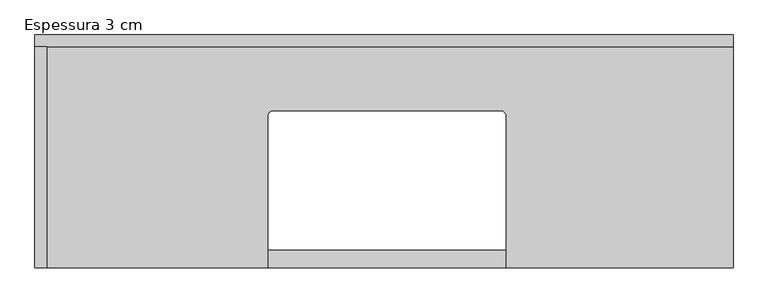
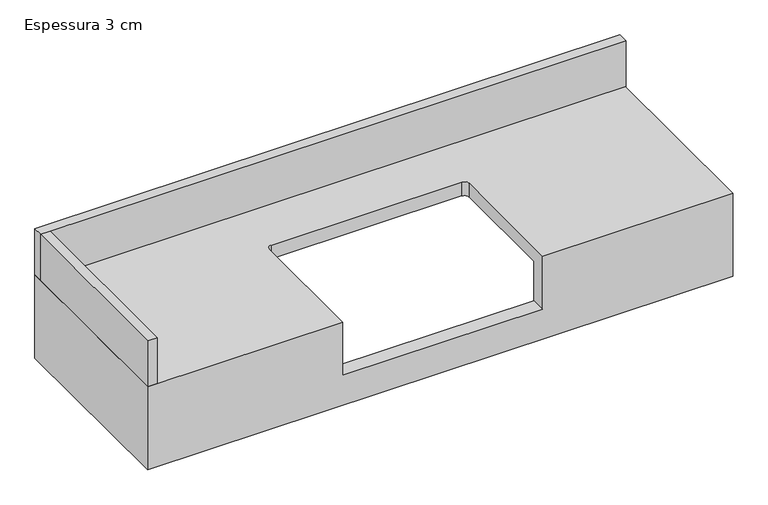
"""IFC4 building model written with IfcOpenShell, lengths in millimetres: furniture geometry, CC_BANCADA BANHEIRO COM CUBA_CANTO RETO : Espessura 3 cm."""

import ifcopenshell
import ifcopenshell.guid

model = None  # the IFC model being written
_history = None  # IfcOwnerHistory: only IFC2X3 demands one
_inside = {}  # id of a spatial element -> (the spatial element, [elements in it])
_under = {}  # id of a project, library or spatial element -> (it, [spatial elements below it])
_declared = {}  # id of a project -> (the project, [libraries it declares])
_typed = {}  # id of a type object -> (the type object, [elements of that type])
_made_of = {}  # id of a material, layer set ... -> (it, [elements and type objects made of it])


def new_model(schema):
    """Start an empty IFC model of exactly this schema.

    Asked for "IFC4X3", IfcOpenShell would pick the latest addendum, in which some entities
    have other attributes; the version numbers below select the first issue.
    IFC2X3 requires an IfcOwnerHistory on every rooted entity: one is made here for all.
    """
    global model, _history
    if schema == "IFC4X3":
        model = ifcopenshell.file(schema_version=(4, 3, 0, 0))
    else:
        model = ifcopenshell.file(schema=schema)
    _inside.clear()
    _under.clear()
    _declared.clear()
    _typed.clear()
    _made_of.clear()
    _history = None
    if model.schema == "IFC2X3":
        org = make("IfcOrganization", Name="unknown")
        user = make(
            "IfcPersonAndOrganization",
            ThePerson=make("IfcPerson", FamilyName="unknown"),
            TheOrganization=org,
        )
        app = make(
            "IfcApplication",
            ApplicationDeveloper=org,
            Version="unknown",
            ApplicationFullName="unknown",
            ApplicationIdentifier="unknown",
        )
        _history = make(
            "IfcOwnerHistory",
            OwningUser=user,
            OwningApplication=app,
            ChangeAction="ADDED",
            CreationDate=0,
        )
    return model


def make(cls, **values):
    """One entity of the class cls with the attributes given. An attribute that is None is left unset."""
    return model.create_entity(
        cls, **{name: value for name, value in values.items() if value is not None}
    )


def rooted(cls, **values):
    """An entity with a GlobalId (a new one), such as an element, a storey or a relation."""
    return make(cls, GlobalId=ifcopenshell.guid.new(), OwnerHistory=_history, **values)


def si_unit(unit_type, name, prefix=None):
    """IfcSIUnit, for example si_unit("LENGTHUNIT", "METRE", prefix="MILLI")."""
    return make("IfcSIUnit", UnitType=unit_type, Prefix=prefix, Name=name)


def assignment(units):
    """IfcUnitAssignment: the units of a project."""
    return None if units is None else make("IfcUnitAssignment", Units=units)


def point(xyz):
    """IfcCartesianPoint."""
    return None if xyz is None else make("IfcCartesianPoint", Coordinates=xyz)


def direction(xyz):
    """IfcDirection."""
    return None if xyz is None else make("IfcDirection", DirectionRatios=xyz)


def frame(location, z_axis=None, x_axis=None):
    """IfcAxis2Placement3D, a coordinate frame: its origin and axes. An axis left out is left unset."""
    return make(
        "IfcAxis2Placement3D",
        Location=point(location),
        Axis=direction(z_axis),
        RefDirection=direction(x_axis),
    )


def origin():
    """The frame at (0, 0, 0) with its axes left unset."""
    return frame((0.0, 0.0, 0.0))


def place(relative_to, where):
    """IfcLocalPlacement: puts the frame where relative to a parent placement (None: the world)."""
    return make(
        "IfcLocalPlacement", PlacementRelTo=relative_to, RelativePlacement=where
    )


def context(
    kind, dimensions, precision=None, world=None, true_north=None, identifier=None
):
    """IfcGeometricRepresentationContext, for example the 3D "Model" context."""
    return make(
        "IfcGeometricRepresentationContext",
        ContextIdentifier=identifier,
        ContextType=kind,
        CoordinateSpaceDimension=dimensions,
        Precision=precision,
        WorldCoordinateSystem=world,
        TrueNorth=true_north,
    )


def project(units=None, contexts=None):
    """IfcProject with its units and contexts."""
    return rooted(
        "IfcProject",
        Name="project",
        RepresentationContexts=contexts,
        UnitsInContext=assignment(units),
    )


def spatial(cls, under=None, at=None, **own):
    """A site, building, storey or space (cls), placed at a placement, below another one or the project."""
    s = rooted(cls, ObjectPlacement=at, **own)
    if under is not None:
        _under.setdefault(under.id(), (under, []))[1].append(s)
    return s


def polyline(points):
    """IfcPolyline through the points."""
    return make("IfcPolyline", Points=[point(p) for p in points])


def circle_curve(where, radius):
    """IfcCircle in the frame where."""
    return make("IfcCircle", Position=where, Radius=radius)


def outline(outer, holes=None, kind="AREA"):
    """IfcArbitraryClosedProfileDef: a profile drawn as a closed curve; with holes, ...WithVoids."""
    if holes is None:
        return make("IfcArbitraryClosedProfileDef", ProfileType=kind, OuterCurve=outer)
    return make(
        "IfcArbitraryProfileDefWithVoids",
        ProfileType=kind,
        OuterCurve=outer,
        InnerCurves=holes,
    )


def extrude(swept, where, along, depth):
    """IfcExtrudedAreaSolid: the profile swept, set in the frame where, extruded along a direction by depth."""
    return make(
        "IfcExtrudedAreaSolid",
        SweptArea=swept,
        Position=where,
        ExtrudedDirection=direction(along),
        Depth=depth,
    )


def shape(context_of_items, identifier, shape_type, items):
    """IfcShapeRepresentation: the items that make up one representation, for example the "Body"."""
    return make(
        "IfcShapeRepresentation",
        ContextOfItems=context_of_items,
        RepresentationIdentifier=identifier,
        RepresentationType=shape_type,
        Items=items,
    )


def source(mapping_origin, context_of_items, identifier, shape_type, items):
    """IfcRepresentationMap: a shape defined once, which mapped items show again and again."""
    return make(
        "IfcRepresentationMap",
        MappingOrigin=mapping_origin,
        MappedRepresentation=shape(context_of_items, identifier, shape_type, items),
    )


def transform(
    local_origin,
    x_axis=None,
    y_axis=None,
    z_axis=None,
    scale=None,
    scale2=None,
    scale3=None,
    uniform=True,
):
    """IfcCartesianTransformationOperator3D, or its non-uniform kind. x_axis, y_axis, z_axis: its Axis1, 2, 3."""
    if uniform:
        return make(
            "IfcCartesianTransformationOperator3D",
            Axis1=direction(x_axis),
            Axis2=direction(y_axis),
            LocalOrigin=point(local_origin),
            Scale=scale,
            Axis3=direction(z_axis),
        )
    return make(
        "IfcCartesianTransformationOperator3DnonUniform",
        Axis1=direction(x_axis),
        Axis2=direction(y_axis),
        LocalOrigin=point(local_origin),
        Scale=scale,
        Axis3=direction(z_axis),
        Scale2=scale2,
        Scale3=scale3,
    )


def mapped(mapping_source, mapping_target):
    """IfcMappedItem: shows the shape of a source again, moved by a transform."""
    return make(
        "IfcMappedItem", MappingSource=mapping_source, MappingTarget=mapping_target
    )


def made_of(thing, what):
    """Note that an element or type object is made of a material, layer set ...; save() writes the relation."""
    if what is not None:
        _made_of.setdefault(what.id(), (what, []))[1].append(thing)
    return thing


def element(
    cls,
    number,
    at=None,
    inside=None,
    cuts=None,
    type_object=None,
    material=None,
    context=None,
    identifier="Body",
    shape_type=None,
    held_by="IfcProductDefinitionShape",
    body=None,
    shapes=None,
    **own,
):
    """One element of the class cls, such as IfcWall. Its Tag is "e" and its number.

    at: its placement. inside: the storey or other place that contains it. cuts: it is an
    opening in that element (IfcRelVoidsElement). A single representation is given by context,
    identifier, shape_type and body (its items); several are given by shapes. held_by: the class
    of the entity that holds the representations. save() writes the other relations.
    """
    e = rooted(cls, Tag="e%d" % number, ObjectPlacement=at, **own)
    if body is not None:
        shapes = [shape(context, identifier, shape_type, body)]
    if shapes is not None:
        e.Representation = make(held_by, Representations=shapes)
    if inside is not None:
        _inside.setdefault(inside.id(), (inside, []))[1].append(e)
    if cuts is not None:
        rooted(
            "IfcRelVoidsElement", RelatingBuildingElement=cuts, RelatedOpeningElement=e
        )
    if type_object is not None:
        _typed.setdefault(type_object.id(), (type_object, []))[1].append(e)
    return made_of(e, material)


def aggregate(whole, parts):
    """IfcRelAggregates: a whole, such as a stair, and the parts it consists of."""
    return rooted("IfcRelAggregates", RelatingObject=whole, RelatedObjects=parts)


def save(model, path):
    """Write the relations noted so far, then the file.

    IfcRelAggregates (storeys below a building ...), IfcRelContainedInSpatialStructure (elements
    in a storey), IfcRelDefinesByType, IfcRelAssociatesMaterial and IfcRelDeclares: one each for
    every whole, place, type object, material and project.
    """
    for whole, parts in _under.values():
        aggregate(whole, parts)
    for where, things in _inside.values():
        rooted(
            "IfcRelContainedInSpatialStructure",
            RelatedElements=things,
            RelatingStructure=where,
        )
    for kind, things in _typed.values():
        rooted("IfcRelDefinesByType", RelatedObjects=things, RelatingType=kind)
    for what, things in _made_of.values():
        rooted("IfcRelAssociatesMaterial", RelatedObjects=things, RelatingMaterial=what)
    for by, libraries in _declared.values():
        rooted("IfcRelDeclares", RelatingContext=by, RelatedDefinitions=libraries)
    model.write(path)


def plane_surface(at):
    """IfcPlane: the flat surface through the origin of the frame at, square to its z axis."""
    return make("IfcPlane", Position=at)


def revolved_surface(curve, axis_point, axis_direction):
    """IfcSurfaceOfRevolution: the curve turned about the line through axis_point along axis_direction."""
    return make(
        "IfcSurfaceOfRevolution",
        SweptCurve=make("IfcArbitraryOpenProfileDef", ProfileType="CURVE", Curve=curve),
        AxisPosition=make("IfcAxis1Placement", Location=point(axis_point), Axis=direction(axis_direction)),
    )


def advanced_brep(points, edges, surfaces, faces):
    """IfcAdvancedBrep: a solid bounded by faces that lie on surfaces and meet in shared edges.

    An edge is (start, end): straight between two places in points (the first is 0);
    or (start, end, curve); or (start, end, curve, False) where it runs against its curve.
    A face is (place in surfaces, loops), or (place, loops, False) where it looks against
    its surface's normal. A loop lists edges by number (the first is 1), with a minus sign
    where the edge is run from its end to its start. The first loop is the outer one.
    """
    corners = [point(p) for p in points]
    vertices = [make("IfcVertexPoint", VertexGeometry=c) for c in corners]
    made = []
    for start, end, *more in edges:
        made.append(
            make(
                "IfcEdgeCurve",
                EdgeStart=vertices[start],
                EdgeEnd=vertices[end],
                EdgeGeometry=more[0] if more else make("IfcPolyline", Points=[corners[start], corners[end]]),
                SameSense=more[1] if len(more) > 1 else True,
            )
        )
    hull = []
    for where, loops, *sense in faces:
        bounds = []
        for j, loop in enumerate(loops):
            ring = [make("IfcOrientedEdge", EdgeElement=made[abs(k) - 1], Orientation=k > 0) for k in loop]
            bounds.append(
                make(
                    "IfcFaceOuterBound" if j == 0 else "IfcFaceBound",
                    Bound=make("IfcEdgeLoop", EdgeList=ring),
                    Orientation=True,
                )
            )
        hull.append(make("IfcAdvancedFace", Bounds=bounds, FaceSurface=surfaces[where], SameSense=sense[0] if sense else True))
    return make("IfcAdvancedBrep", Outer=make("IfcClosedShell", CfsFaces=hull))


def espessura_3_cm_a8edac31(model_context):
    return source(origin(), model_context, "Body", "SolidModel", [
        advanced_brep(
        [(750.0, 300.0, 860.0), (-450.0, 300.0, 860.0), (-450.0, -100.0, 860.0), (-50.0, -100.0, 860.0), (-50.0, 160.0, 860.0), (-40.0, 170.0, 860.0), (350.0, 170.0, 860.0), (360.0, 160.0, 860.0), (360.0, -100.0, 860.0), (750.0, -100.0, 860.0), (750.0, 300.0, 680.0), (720.0, 300.0, 680.0), (720.0, 300.0, 830.0), (-420.0, 300.0, 830.0), (-420.0, 300.0, 680.0), (-450.0, 300.0, 680.0), (-450.0, -100.0, 680.0), (750.0, -100.0, 680.0), (360.0, -100.0, 745.0), (-50.0, -100.0, 745.0), (720.0, -70.0, 830.0), (360.0, -70.0, 830.0), (360.0, 160.0, 830.0), (350.0, 170.0, 830.0), (-40.0, 170.0, 830.0), (-50.0, 160.0, 830.0), (-50.0, -70.0, 830.0), (-420.0, -70.0, 830.0), (-420.0, -70.0, 680.0), (-50.0, -70.0, 745.0), (360.0, -70.0, 745.0), (720.0, -70.0, 680.0)],
        [
            (0, 1),
            (1, 2),
            (2, 3),
            (3, 4),
            (4, 5, circle_curve(frame((-40.0, 160.0, 860.0), z_axis=(0.0, 0.0, -1.0), x_axis=(0.0, 1.0, 0.0)), 10.0)),
            (5, 6),
            (6, 7, circle_curve(frame((350.0, 160.0, 860.0), z_axis=(0.0, 0.0, -1.0), x_axis=(0.0, 1.0, 0.0)), 10.0)),
            (7, 8),
            (8, 9),
            (9, 0),
            (0, 10),
            (10, 11),
            (11, 12),
            (12, 13),
            (13, 14),
            (14, 15),
            (15, 1),
            (15, 16),
            (16, 2),
            (16, 17),
            (17, 9),
            (8, 18),
            (18, 19),
            (19, 3),
            (17, 10),
            (12, 20),
            (20, 21),
            (21, 22),
            (22, 23, circle_curve(frame((350.0, 160.0, 830.0), z_axis=(0.0, 0.0, 1.0), x_axis=(0.0, 1.0, 0.0)), 10.0)),
            (23, 24),
            (24, 25, circle_curve(frame((-40.0, 160.0, 830.0), z_axis=(0.0, 0.0, 1.0), x_axis=(0.0, 1.0, 0.0)), 10.0)),
            (25, 26),
            (26, 27),
            (27, 13),
            (27, 28),
            (28, 14),
            (26, 29),
            (29, 30),
            (30, 21),
            (20, 31),
            (31, 28),
            (11, 31),
            (5, 24),
            (23, 6),
            (18, 30),
            (29, 19),
            (4, 25),
            (7, 22),
        ],
        [
            plane_surface(frame((-450.0, 300.0, 860.0), z_axis=(0.0, 0.0, 1.0), x_axis=(-1.0, 0.0, 0.0))),
            plane_surface(frame((750.0, 300.0, 860.0), z_axis=(0.0, 1.0, 0.0), x_axis=(0.0, 0.0, -1.0))),
            plane_surface(frame((-450.0, 300.0, 860.0), z_axis=(-1.0, 0.0, 0.0), x_axis=(0.0, 0.0, -1.0))),
            plane_surface(frame((-450.0, -100.0, 860.0), z_axis=(0.0, -1.0, 0.0), x_axis=(0.0, 0.0, -1.0))),
            plane_surface(frame((750.0, -100.0, 860.0), z_axis=(1.0, 0.0, 0.0), x_axis=(0.0, 0.0, -1.0))),
            plane_surface(frame((-420.0, 300.0, 830.0), z_axis=(0.0, 0.0, -1.0), x_axis=(-1.0, 0.0, 0.0))),
            plane_surface(frame((-420.0, 300.0, 830.0), z_axis=(1.0, 0.0, 0.0), x_axis=(0.0, 0.0, -1.0))),
            plane_surface(frame((-420.0, -70.0, 830.0), z_axis=(0.0, 1.0, 0.0), x_axis=(0.0, 0.0, -1.0))),
            plane_surface(frame((720.0, -70.0, 830.0), z_axis=(-1.0, 0.0, 0.0), x_axis=(0.0, 0.0, -1.0))),
            plane_surface(frame((750.0, -100.0, 680.0), z_axis=(0.0, 0.0, -1.0), x_axis=(0.0, 1.0, 0.0))),
            plane_surface(frame((-40.0, 170.0, 745.0), z_axis=(0.0, -1.0, 0.0), x_axis=(0.0, 0.0, 1.0))),
            plane_surface(frame((350.0, 170.0, 745.0), z_axis=(0.0, 0.0, 1.0), x_axis=(1.0, 0.0, 0.0))),
            revolved_surface(polyline([(-40.0, 170.0, 830.0), (-40.0, 170.0, 860.0)]), (-40.0, 160.0, 900.0), (0.0, 0.0, -1.0)),
            plane_surface(frame((-50.0, -230.0, 745.0), z_axis=(1.0, 0.0, 0.0), x_axis=(0.0, 0.0, 1.0))),
            plane_surface(frame((360.0, 160.0, 745.0), z_axis=(-1.0, 0.0, 0.0), x_axis=(0.0, 0.0, 1.0))),
            revolved_surface(polyline([(350.0, 170.0, 830.0), (350.0, 170.0, 860.0)]), (350.0, 160.0, 900.0), (0.0, 0.0, -1.0)),
        ],
        [
            (0, [[1, 2, 3, 4, 5, 6, 7, 8, 9, 10]]),
            (1, [[-1, 11, 12, 13, 14, 15, 16, 17]]),
            (2, [[-2, -17, 18, 19]]),
            (3, [[-3, -19, 20, 21, -9, 22, 23, 24]]),
            (4, [[-10, -21, 25, -11]]),
            (5, [[26, 27, 28, 29, 30, 31, 32, 33, 34, -14]]),
            (6, [[-34, 35, 36, -15]]),
            (7, [[-33, 37, 38, 39, -27, 40, 41, -35]]),
            (8, [[-26, -13, 42, -40]]),
            (9, [[-12, -25, -20, -18, -16, -36, -41, -42]]),
            (10, [[-6, 43, -30, 44]]),
            (11, [[-23, 45, -38, 46]]),
            (12, [[-5, 47, -31, -43]]),
            (13, [[-4, -24, -46, -37, -32, -47]]),
            (14, [[-8, 48, -28, -39, -45, -22]]),
            (15, [[-7, -44, -29, -48]]),
        ],
    ),
        extrude(outline(polyline([(-430.0, -100.0), (-450.0, -100.0), (-450.0, 280.0), (-430.0, 280.0), (-430.0, -100.0)])), frame((0.0, 0.0, 860.0), z_axis=(0.0, 0.0, 1.0), x_axis=(1.0, 0.0, 0.0)), (0.0, 0.0, 1.0), 100.0),
        extrude(outline(polyline([(750.0, 300.0), (750.0, 280.0), (-450.0, 280.0), (-450.0, 300.0), (750.0, 300.0)])), frame((0.0, 0.0, 860.0), z_axis=(0.0, 0.0, 1.0), x_axis=(1.0, 0.0, 0.0)), (0.0, 0.0, 1.0), 100.0),
    ])


if __name__ == "__main__":
    model = new_model("IFC4")
    model_context = context("Model", 3, world=origin())
    ifc_project = project(units=[si_unit("LENGTHUNIT", "METRE", prefix="MILLI")], contexts=[model_context])
    site = spatial("IfcSite", under=ifc_project)
    building = spatial("IfcBuilding", under=site)
    placement = place(None, origin())
    espessura_3_cm_shape = espessura_3_cm_a8edac31(model_context)
    element("IfcFurniture", 1, ObjectType="CC_BANCADA BANHEIRO COM CUBA_CANTO RETO : Espessura 3 cm", at=placement, inside=building, context=model_context, shape_type="MappedRepresentation", body=[
        mapped(espessura_3_cm_shape, transform((0.0, 0.0, 0.0), x_axis=(1.0, 0.0, 0.0), y_axis=(0.0, 1.0, 0.0), z_axis=(0.0, 0.0, 1.0))),
    ])
    save(model, "model.ifc")

# Revit data of these elements
# Type "CC_BANCADA BANHEIRO COM CUBA_CANTO RETO : Espessura 3 cm"
#   Uso HS [instance default] = ""
#   h TESTEIRA AUX [instance default] = 0.15 m
#   Altura testeira [instance default] = 0.15 m
#   Altura rodapia [instance default] = 0.10 m
#   Espessura rodapia [instance default] = 0.02 m
#   Prof/2 [instance default] = 0.20 m
#   Offset cuba esquerda [instance default] = 0.40 m
#   Depth [instance default] = 1.20 m
#   Width [instance default] = 0.40 m
#   Espessura bancada = 0.03 m
#   Comprimento [instance default] = 1.20 m
#   Height [instance default] = 0.86 m
#   Testeira [instance default] = yes
#   Rodapia fundo [instance default] = no
#   Rodapia esquerda [instance default] = no
#   Rodapia direita [instance default] = no
#   Material porta-toalha [instance default] = .CROMADO
#   Material hidráulico [instance default] = .CROMADO
#   Material cuba [instance default] = .PORCELANA BRANCA
#   Material bancada [instance default] = .GRANITO_BRANCO_ITAUNAS
#   Assembly Code = ""
# Element 1 (IfcFurniture, "CC_BANCADA BANHEIRO COM CUBA_CANTO RETO : Espessura 3 cm")
#   Uso HS = "BANHO SUÍTE 2"
#   Rodapia fundo = yes
#   Rodapia esquerda = yes
#   Materials on its faces: ".GRANITO_BRANCO_ITAUNAS"
# Materials
#   ".CROMADO": class "CC_METAIS", colour RGB 211 223 226, transparency 0, Cost = 0
#   ".PORCELANA BRANCA": class "CC_PORCELANA", colour RGB 230 230 230, transparency 0, Cost = 0
#   ".GRANITO_BRANCO_ITAUNAS": class ".CC_PEDRA REVEST.", colour RGB 202 195 174, transparency 0, Description = "Revestimento em granito", Cost = 0
